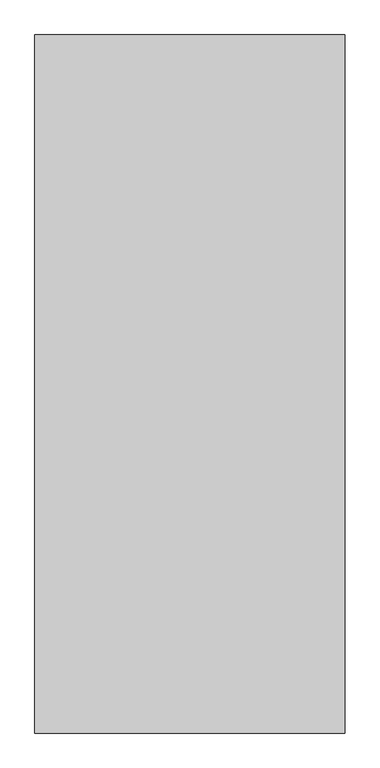
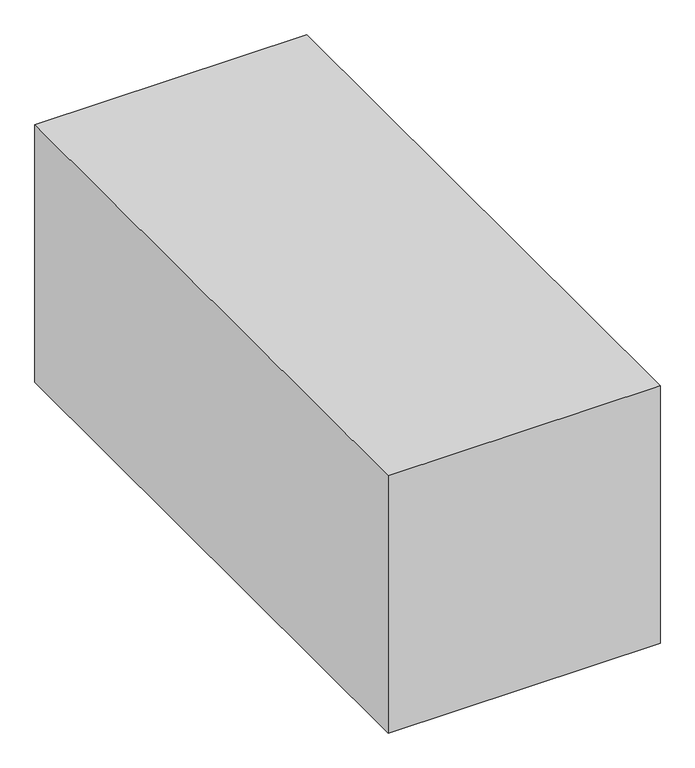
"""IFC4 building model written with IfcOpenShell, lengths in millimetres: proxy geometry, Space Planning Box_hec : Space Planning Box_hec."""

from ifc_helpers import new_model, si_unit, origin, origin_with_axes, place, context, project, spatial, polyline, outline, extrude, source, transform, mapped, element, save


def generic_models_73802227(model_context):
    return source(origin(), model_context, "Body", "SweptSolid", [
        extrude(outline(polyline([(2000.0, 4500.0), (2000.0, -4500.0), (-2000.0, -4500.0), (-2000.0, 4500.0), (2000.0, 4500.0)])), origin_with_axes(), (0.0, 0.0, 1.0), 4000.0),
    ])


if __name__ == "__main__":
    model = new_model("IFC4")
    model_context = context("Model", 3, world=origin())
    ifc_project = project(units=[si_unit("LENGTHUNIT", "METRE", prefix="MILLI")], contexts=[model_context])
    site = spatial("IfcSite", under=ifc_project)
    building = spatial("IfcBuilding", under=site)
    placement = place(None, origin())
    generic_models_shape = generic_models_73802227(model_context)
    element("IfcBuildingElementProxy", 1, Name="Space Planning Box_hec : Space Planning Box_hec", ObjectType="Space Planning Box_hec : Space Planning Box_hec", at=placement, inside=building, context=model_context, shape_type="MappedRepresentation", body=[
        mapped(generic_models_shape, transform((0.0, 0.0, 0.0), x_axis=(1.0, 0.0, 0.0), y_axis=(0.0, 1.0, 0.0), z_axis=(0.0, 0.0, 1.0))),
    ])
    save(model, "model.ifc")

# Revit data of these elements
# Type "Space Planning Box_hec : Space Planning Box_hec"
#   Type Comments = "..."
#   Room Name [instance default] = "?"
#   Interior Finish [instance default] = ""
#   Exterior Finish [instance default] = ""
#   Department [instance default] = ""
#   Assembly Code = "..."
#   Width [instance default] = 1524 mm
#   Program Area [instance default] = 0 m²
#   Length [instance default] = 1524 mm
#   Height [instance default] = 1524 mm
#   Area [instance default] = 2.32258 m²
#   Fill Color [instance default] = Cyan
#   Default Elevation = 0
# Element 1 (IfcBuildingElementProxy, "Space Planning Box_hec : Space Planning Box_hec")
#   Room Name = "Stairway"
#   Interior Finish = "IF2"
#   Exterior Finish = "EF1"
#   Department = "EL"
#   Width = 4000 mm
#   Program Area = 36 m²
#   Length = 9000 mm
#   Height = 4000 mm
#   Area = 36 m²
#   Fill Color = Blue
#   Materials on its faces: "Blue"
# Materials
#   "Cyan": class "Generic", colour RGB 0 255 255, transparency 0.2, Cost = 0
#   "Blue": class "Generic", colour RGB 0 0 255, transparency 0.2, Cost = 0
